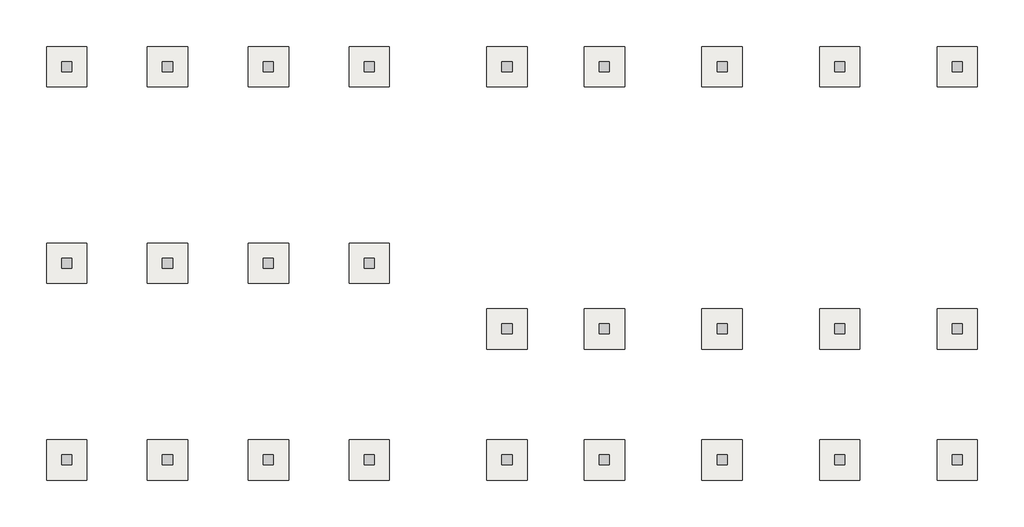
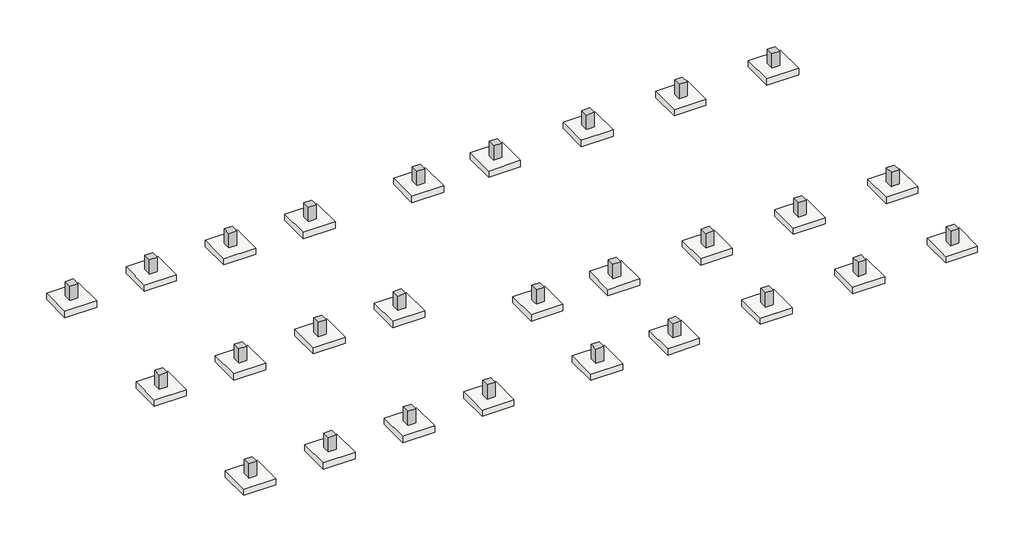
# Not in any storey: 27 columns, 27 slabs.
"""IFC4 building model written with IfcOpenShell, lengths in millimetres."""

import ifcopenshell
import ifcopenshell.guid

model = None  # the IFC model being written
_history = None  # IfcOwnerHistory: only IFC2X3 demands one
_inside = {}  # id of a spatial element -> (the spatial element, [elements in it])
_under = {}  # id of a project, library or spatial element -> (it, [spatial elements below it])
_declared = {}  # id of a project -> (the project, [libraries it declares])
_typed = {}  # id of a type object -> (the type object, [elements of that type])
_made_of = {}  # id of a material, layer set ... -> (it, [elements and type objects made of it])


def new_model(schema):
    """Start an empty IFC model of exactly this schema.

    Asked for "IFC4X3", IfcOpenShell would pick the latest addendum, in which some entities
    have other attributes; the version numbers below select the first issue.
    IFC2X3 requires an IfcOwnerHistory on every rooted entity: one is made here for all.
    """
    global model, _history
    if schema == "IFC4X3":
        model = ifcopenshell.file(schema_version=(4, 3, 0, 0))
    else:
        model = ifcopenshell.file(schema=schema)
    _inside.clear()
    _under.clear()
    _declared.clear()
    _typed.clear()
    _made_of.clear()
    _history = None
    if model.schema == "IFC2X3":
        org = make("IfcOrganization", Name="unknown")
        user = make(
            "IfcPersonAndOrganization",
            ThePerson=make("IfcPerson", FamilyName="unknown"),
            TheOrganization=org,
        )
        app = make(
            "IfcApplication",
            ApplicationDeveloper=org,
            Version="unknown",
            ApplicationFullName="unknown",
            ApplicationIdentifier="unknown",
        )
        _history = make(
            "IfcOwnerHistory",
            OwningUser=user,
            OwningApplication=app,
            ChangeAction="ADDED",
            CreationDate=0,
        )
    return model


def make(cls, **values):
    """One entity of the class cls with the attributes given. An attribute that is None is left unset."""
    return model.create_entity(
        cls, **{name: value for name, value in values.items() if value is not None}
    )


def rooted(cls, **values):
    """An entity with a GlobalId (a new one), such as an element, a storey or a relation."""
    return make(cls, GlobalId=ifcopenshell.guid.new(), OwnerHistory=_history, **values)


def si_unit(unit_type, name, prefix=None):
    """IfcSIUnit, for example si_unit("LENGTHUNIT", "METRE", prefix="MILLI")."""
    return make("IfcSIUnit", UnitType=unit_type, Prefix=prefix, Name=name)


def assignment(units):
    """IfcUnitAssignment: the units of a project."""
    return None if units is None else make("IfcUnitAssignment", Units=units)


def point(xyz):
    """IfcCartesianPoint."""
    return None if xyz is None else make("IfcCartesianPoint", Coordinates=xyz)


def direction(xyz):
    """IfcDirection."""
    return None if xyz is None else make("IfcDirection", DirectionRatios=xyz)


def frame(location, z_axis=None, x_axis=None):
    """IfcAxis2Placement3D, a coordinate frame: its origin and axes. An axis left out is left unset."""
    return make(
        "IfcAxis2Placement3D",
        Location=point(location),
        Axis=direction(z_axis),
        RefDirection=direction(x_axis),
    )


def origin():
    """The frame at (0, 0, 0) with its axes left unset."""
    return frame((0.0, 0.0, 0.0))


def place(relative_to, where):
    """IfcLocalPlacement: puts the frame where relative to a parent placement (None: the world)."""
    return make(
        "IfcLocalPlacement", PlacementRelTo=relative_to, RelativePlacement=where
    )


def context(
    kind, dimensions, precision=None, world=None, true_north=None, identifier=None
):
    """IfcGeometricRepresentationContext, for example the 3D "Model" context."""
    return make(
        "IfcGeometricRepresentationContext",
        ContextIdentifier=identifier,
        ContextType=kind,
        CoordinateSpaceDimension=dimensions,
        Precision=precision,
        WorldCoordinateSystem=world,
        TrueNorth=true_north,
    )


def project(units=None, contexts=None):
    """IfcProject with its units and contexts."""
    return rooted(
        "IfcProject",
        Name="project",
        RepresentationContexts=contexts,
        UnitsInContext=assignment(units),
    )


def spatial(cls, under=None, at=None, **own):
    """A site, building, storey or space (cls), placed at a placement, below another one or the project."""
    s = rooted(cls, ObjectPlacement=at, **own)
    if under is not None:
        _under.setdefault(under.id(), (under, []))[1].append(s)
    return s


def polyline(points):
    """IfcPolyline through the points."""
    return make("IfcPolyline", Points=[point(p) for p in points])


def outline(outer, holes=None, kind="AREA"):
    """IfcArbitraryClosedProfileDef: a profile drawn as a closed curve; with holes, ...WithVoids."""
    if holes is None:
        return make("IfcArbitraryClosedProfileDef", ProfileType=kind, OuterCurve=outer)
    return make(
        "IfcArbitraryProfileDefWithVoids",
        ProfileType=kind,
        OuterCurve=outer,
        InnerCurves=holes,
    )


def extrude(swept, where, along, depth):
    """IfcExtrudedAreaSolid: the profile swept, set in the frame where, extruded along a direction by depth."""
    return make(
        "IfcExtrudedAreaSolid",
        SweptArea=swept,
        Position=where,
        ExtrudedDirection=direction(along),
        Depth=depth,
    )


def shape(context_of_items, identifier, shape_type, items):
    """IfcShapeRepresentation: the items that make up one representation, for example the "Body"."""
    return make(
        "IfcShapeRepresentation",
        ContextOfItems=context_of_items,
        RepresentationIdentifier=identifier,
        RepresentationType=shape_type,
        Items=items,
    )


def source(mapping_origin, context_of_items, identifier, shape_type, items):
    """IfcRepresentationMap: a shape defined once, which mapped items show again and again."""
    return make(
        "IfcRepresentationMap",
        MappingOrigin=mapping_origin,
        MappedRepresentation=shape(context_of_items, identifier, shape_type, items),
    )


def transform(
    local_origin,
    x_axis=None,
    y_axis=None,
    z_axis=None,
    scale=None,
    scale2=None,
    scale3=None,
    uniform=True,
):
    """IfcCartesianTransformationOperator3D, or its non-uniform kind. x_axis, y_axis, z_axis: its Axis1, 2, 3."""
    if uniform:
        return make(
            "IfcCartesianTransformationOperator3D",
            Axis1=direction(x_axis),
            Axis2=direction(y_axis),
            LocalOrigin=point(local_origin),
            Scale=scale,
            Axis3=direction(z_axis),
        )
    return make(
        "IfcCartesianTransformationOperator3DnonUniform",
        Axis1=direction(x_axis),
        Axis2=direction(y_axis),
        LocalOrigin=point(local_origin),
        Scale=scale,
        Axis3=direction(z_axis),
        Scale2=scale2,
        Scale3=scale3,
    )


def mapped(mapping_source, mapping_target):
    """IfcMappedItem: shows the shape of a source again, moved by a transform."""
    return make(
        "IfcMappedItem", MappingSource=mapping_source, MappingTarget=mapping_target
    )


def made_of(thing, what):
    """Note that an element or type object is made of a material, layer set ...; save() writes the relation."""
    if what is not None:
        _made_of.setdefault(what.id(), (what, []))[1].append(thing)
    return thing


def element(
    cls,
    number,
    at=None,
    inside=None,
    cuts=None,
    type_object=None,
    material=None,
    context=None,
    identifier="Body",
    shape_type=None,
    held_by="IfcProductDefinitionShape",
    body=None,
    shapes=None,
    **own,
):
    """One element of the class cls, such as IfcWall. Its Tag is "e" and its number.

    at: its placement. inside: the storey or other place that contains it. cuts: it is an
    opening in that element (IfcRelVoidsElement). A single representation is given by context,
    identifier, shape_type and body (its items); several are given by shapes. held_by: the class
    of the entity that holds the representations. save() writes the other relations.
    """
    e = rooted(cls, Tag="e%d" % number, ObjectPlacement=at, **own)
    if body is not None:
        shapes = [shape(context, identifier, shape_type, body)]
    if shapes is not None:
        e.Representation = make(held_by, Representations=shapes)
    if inside is not None:
        _inside.setdefault(inside.id(), (inside, []))[1].append(e)
    if cuts is not None:
        rooted(
            "IfcRelVoidsElement", RelatingBuildingElement=cuts, RelatedOpeningElement=e
        )
    if type_object is not None:
        _typed.setdefault(type_object.id(), (type_object, []))[1].append(e)
    return made_of(e, material)


def aggregate(whole, parts):
    """IfcRelAggregates: a whole, such as a stair, and the parts it consists of."""
    return rooted("IfcRelAggregates", RelatingObject=whole, RelatedObjects=parts)


def save(model, path):
    """Write the relations noted so far, then the file.

    IfcRelAggregates (storeys below a building ...), IfcRelContainedInSpatialStructure (elements
    in a storey), IfcRelDefinesByType, IfcRelAssociatesMaterial and IfcRelDeclares: one each for
    every whole, place, type object, material and project.
    """
    for whole, parts in _under.values():
        aggregate(whole, parts)
    for where, things in _inside.values():
        rooted(
            "IfcRelContainedInSpatialStructure",
            RelatedElements=things,
            RelatingStructure=where,
        )
    for kind, things in _typed.values():
        rooted("IfcRelDefinesByType", RelatedObjects=things, RelatingType=kind)
    for what, things in _made_of.values():
        rooted("IfcRelAssociatesMaterial", RelatedObjects=things, RelatingMaterial=what)
    for by, libraries in _declared.values():
        rooted("IfcRelDeclares", RelatingContext=by, RelatedDefinitions=libraries)
    model.write(path)


def foundation_rectangular_non_pile_5fe39465(model_context):
    return source(origin(), model_context, "Body", "SweptSolid", [
        extrude(outline(polyline([(1200.0, 1200.0), (1200.0, -1200.0), (-1200.0, -1200.0), (-1200.0, 1200.0), (1200.0, 1200.0)])), frame((0.0, 0.0, -500.0), z_axis=(0.0, 0.0, 1.0), x_axis=(1.0, 0.0, 0.0)), (0.0, 0.0, 1.0), 500.0),
    ])


model = new_model("IFC4")

# Units and contexts
model_context = context("Model", 3, world=origin())
ifc_project = project(units=[si_unit("LENGTHUNIT", "METRE", prefix="MILLI")], contexts=[model_context])

# Site, building
site = spatial("IfcSite", under=ifc_project)
building = spatial("IfcBuilding", under=site)

# Columns
placement = place(None, origin())
element("IfcColumn", 1, ObjectType="RC_Column_Rectangular : H_SC_AR_S15_UG PED_W600xL600_Bit_Anchor", at=placement, inside=building, context=model_context, shape_type="SweptSolid", body=[
    extrude(outline(polyline([(300.0, 12499.5208589), (300.0, 11899.5208589), (-300.0, 11899.5208589), (-300.0, 12499.5208589), (300.0, 12499.5208589)])), frame((0.0, 0.0, -1000.0381366), z_axis=(0.0, 0.0, 1.0), x_axis=(1.0, 0.0, 0.0)), (0.0, 0.0, 1.0), 1150.0),
])
element("IfcColumn", 2, ObjectType="RC_Column_Rectangular : H_SC_AR_S15_UG PED_W600xL600_Bit_Anchor", at=placement, inside=building, context=model_context, shape_type="SweptSolid", body=[
    extrude(outline(polyline([(6300.0, 12499.5208589), (6300.0, 11899.5208589), (5700.0, 11899.5208589), (5700.0, 12499.5208589), (6300.0, 12499.5208589)])), frame((0.0, 0.0, -1000.0381366), z_axis=(0.0, 0.0, 1.0), x_axis=(1.0, 0.0, 0.0)), (0.0, 0.0, 1.0), 1150.0),
])
element("IfcColumn", 3, ObjectType="RC_Column_Rectangular : H_SC_AR_S15_UG PED_W600xL600_Bit_Anchor", at=placement, inside=building, context=model_context, shape_type="SweptSolid", body=[
    extrude(outline(polyline([(12300.0, 12499.5208589), (12300.0, 11899.5208589), (11700.0, 11899.5208589), (11700.0, 12499.5208589), (12300.0, 12499.5208589)])), frame((0.0, 0.0, -1000.0381366), z_axis=(0.0, 0.0, 1.0), x_axis=(1.0, 0.0, 0.0)), (0.0, 0.0, 1.0), 1150.0),
])
element("IfcColumn", 4, ObjectType="RC_Column_Rectangular : H_SC_AR_S15_UG PED_W600xL600_Bit_Anchor", at=placement, inside=building, context=model_context, shape_type="SweptSolid", body=[
    extrude(outline(polyline([(18300.0, 12499.5208589), (18300.0, 11899.5208589), (17700.0, 11899.5208589), (17700.0, 12499.5208589), (18300.0, 12499.5208589)])), frame((0.0, 0.0, -1000.0381366), z_axis=(0.0, 0.0, 1.0), x_axis=(1.0, 0.0, 0.0)), (0.0, 0.0, 1.0), 1150.0),
])
element("IfcColumn", 5, ObjectType="RC_Column_Rectangular : H_SC_AR_S15_UG PED_W600xL600_Bit_Anchor", at=placement, inside=building, context=model_context, shape_type="SweptSolid", body=[
    extrude(outline(polyline([(300.0, 24199.5208589), (300.0, 23599.5208589), (-300.0, 23599.5208589), (-300.0, 24199.5208589), (300.0, 24199.5208589)])), frame((0.0, 0.0, -1000.0381366), z_axis=(0.0, 0.0, 1.0), x_axis=(1.0, 0.0, 0.0)), (0.0, 0.0, 1.0), 1150.0),
])
element("IfcColumn", 6, ObjectType="RC_Column_Rectangular : H_SC_AR_S15_UG PED_W600xL600_Bit_Anchor", at=placement, inside=building, context=model_context, shape_type="SweptSolid", body=[
    extrude(outline(polyline([(6300.0, 24199.5208589), (6300.0, 23599.5208589), (5700.0, 23599.5208589), (5700.0, 24199.5208589), (6300.0, 24199.5208589)])), frame((0.0, 0.0, -1000.0381366), z_axis=(0.0, 0.0, 1.0), x_axis=(1.0, 0.0, 0.0)), (0.0, 0.0, 1.0), 1150.0),
])
element("IfcColumn", 7, ObjectType="RC_Column_Rectangular : H_SC_AR_S15_UG PED_W600xL600_Bit_Anchor", at=placement, inside=building, context=model_context, shape_type="SweptSolid", body=[
    extrude(outline(polyline([(12300.0, 24199.5208589), (12300.0, 23599.5208589), (11700.0, 23599.5208589), (11700.0, 24199.5208589), (12300.0, 24199.5208589)])), frame((0.0, 0.0, -1000.0381366), z_axis=(0.0, 0.0, 1.0), x_axis=(1.0, 0.0, 0.0)), (0.0, 0.0, 1.0), 1150.0),
])
element("IfcColumn", 8, ObjectType="RC_Column_Rectangular : H_SC_AR_S15_UG PED_W600xL600_Bit_Anchor", at=placement, inside=building, context=model_context, shape_type="SweptSolid", body=[
    extrude(outline(polyline([(18300.0, 24199.5208589), (18300.0, 23599.5208589), (17700.0, 23599.5208589), (17700.0, 24199.5208589), (18300.0, 24199.5208589)])), frame((0.0, 0.0, -1000.0381366), z_axis=(0.0, 0.0, 1.0), x_axis=(1.0, 0.0, 0.0)), (0.0, 0.0, 1.0), 1150.0),
])
element("IfcColumn", 9, ObjectType="RC_Column_Rectangular : H_SC_AR_S15_UG PED_W600xL600_Bit_Anchor", at=placement, inside=building, context=model_context, shape_type="SweptSolid", body=[
    extrude(outline(polyline([(26500.0, 24199.5208589), (26500.0, 23599.5208589), (25900.0, 23599.5208589), (25900.0, 24199.5208589), (26500.0, 24199.5208589)])), frame((0.0, 0.0, -1000.0381366), z_axis=(0.0, 0.0, 1.0), x_axis=(1.0, 0.0, 0.0)), (0.0, 0.0, 1.0), 1150.0),
])
element("IfcColumn", 10, ObjectType="RC_Column_Rectangular : H_SC_AR_S15_UG PED_W600xL600_Bit_Anchor", at=placement, inside=building, context=model_context, shape_type="SweptSolid", body=[
    extrude(outline(polyline([(32300.0, 24199.5208589), (32300.0, 23599.5208589), (31700.0, 23599.5208589), (31700.0, 24199.5208589), (32300.0, 24199.5208589)])), frame((0.0, 0.0, -1000.0381366), z_axis=(0.0, 0.0, 1.0), x_axis=(1.0, 0.0, 0.0)), (0.0, 0.0, 1.0), 1150.0),
])
element("IfcColumn", 11, ObjectType="RC_Column_Rectangular : H_SC_AR_S15_UG PED_W600xL600_Bit_Anchor", at=placement, inside=building, context=model_context, shape_type="SweptSolid", body=[
    extrude(outline(polyline([(39300.0, 24199.5208589), (39300.0, 23599.5208589), (38700.0, 23599.5208589), (38700.0, 24199.5208589), (39300.0, 24199.5208589)])), frame((0.0, 0.0, -1000.0381366), z_axis=(0.0, 0.0, 1.0), x_axis=(1.0, 0.0, 0.0)), (0.0, 0.0, 1.0), 1150.0),
])
element("IfcColumn", 12, ObjectType="RC_Column_Rectangular : H_SC_AR_S15_UG PED_W600xL600_Bit_Anchor", at=placement, inside=building, context=model_context, shape_type="SweptSolid", body=[
    extrude(outline(polyline([(46300.0, 24199.5208589), (46300.0, 23599.5208589), (45700.0, 23599.5208589), (45700.0, 24199.5208589), (46300.0, 24199.5208589)])), frame((0.0, 0.0, -1000.0381366), z_axis=(0.0, 0.0, 1.0), x_axis=(1.0, 0.0, 0.0)), (0.0, 0.0, 1.0), 1150.0),
])
element("IfcColumn", 13, ObjectType="RC_Column_Rectangular : H_SC_AR_S15_UG PED_W600xL600_Bit_Anchor", at=placement, inside=building, context=model_context, shape_type="SweptSolid", body=[
    extrude(outline(polyline([(53300.0, 24199.5208589), (53300.0, 23599.5208589), (52700.0, 23599.5208589), (52700.0, 24199.5208589), (53300.0, 24199.5208589)])), frame((0.0, 0.0, -1000.0381366), z_axis=(0.0, 0.0, 1.0), x_axis=(1.0, 0.0, 0.0)), (0.0, 0.0, 1.0), 1150.0),
])
element("IfcColumn", 14, ObjectType="RC_Column_Rectangular : H_SC_AR_S15_UG PED_W600xL600_Bit_Anchor", at=placement, inside=building, context=model_context, shape_type="SweptSolid", body=[
    extrude(outline(polyline([(26500.0, 8599.5208589), (26500.0, 7999.5208589), (25900.0, 7999.5208589), (25900.0, 8599.5208589), (26500.0, 8599.5208589)])), frame((0.0, 0.0, -1000.0381366), z_axis=(0.0, 0.0, 1.0), x_axis=(1.0, 0.0, 0.0)), (0.0, 0.0, 1.0), 1150.0),
])
element("IfcColumn", 15, ObjectType="RC_Column_Rectangular : H_SC_AR_S15_UG PED_W600xL600_Bit_Anchor", at=placement, inside=building, context=model_context, shape_type="SweptSolid", body=[
    extrude(outline(polyline([(32300.0, 8599.5208589), (32300.0, 7999.5208589), (31700.0, 7999.5208589), (31700.0, 8599.5208589), (32300.0, 8599.5208589)])), frame((0.0, 0.0, -1000.0381366), z_axis=(0.0, 0.0, 1.0), x_axis=(1.0, 0.0, 0.0)), (0.0, 0.0, 1.0), 1150.0),
])
element("IfcColumn", 16, ObjectType="RC_Column_Rectangular : H_SC_AR_S15_UG PED_W600xL600_Bit_Anchor", at=placement, inside=building, context=model_context, shape_type="SweptSolid", body=[
    extrude(outline(polyline([(39300.0, 8599.5208589), (39300.0, 7999.5208589), (38700.0, 7999.5208589), (38700.0, 8599.5208589), (39300.0, 8599.5208589)])), frame((0.0, 0.0, -1000.0381366), z_axis=(0.0, 0.0, 1.0), x_axis=(1.0, 0.0, 0.0)), (0.0, 0.0, 1.0), 1150.0),
])
element("IfcColumn", 17, ObjectType="RC_Column_Rectangular : H_SC_AR_S15_UG PED_W600xL600_Bit_Anchor", at=placement, inside=building, context=model_context, shape_type="SweptSolid", body=[
    extrude(outline(polyline([(46300.0, 8599.5208589), (46300.0, 7999.5208589), (45700.0, 7999.5208589), (45700.0, 8599.5208589), (46300.0, 8599.5208589)])), frame((0.0, 0.0, -1000.0381366), z_axis=(0.0, 0.0, 1.0), x_axis=(1.0, 0.0, 0.0)), (0.0, 0.0, 1.0), 1150.0),
])
element("IfcColumn", 18, ObjectType="RC_Column_Rectangular : H_SC_AR_S15_UG PED_W600xL600_Bit_Anchor", at=placement, inside=building, context=model_context, shape_type="SweptSolid", body=[
    extrude(outline(polyline([(53300.0, 8599.5208589), (53300.0, 7999.5208589), (52700.0, 7999.5208589), (52700.0, 8599.5208589), (53300.0, 8599.5208589)])), frame((0.0, 0.0, -1000.0381366), z_axis=(0.0, 0.0, 1.0), x_axis=(1.0, 0.0, 0.0)), (0.0, 0.0, 1.0), 1150.0),
])
element("IfcColumn", 19, ObjectType="RC_Column_Rectangular : H_SC_AR_S15_UG PED_W600xL600_Bit_Anchor", at=placement, inside=building, context=model_context, shape_type="SweptSolid", body=[
    extrude(outline(polyline([(300.0, 799.5208589), (300.0, 199.5208589), (-300.0, 199.5208589), (-300.0, 799.5208589), (300.0, 799.5208589)])), frame((0.0, 0.0, -1000.0381366), z_axis=(0.0, 0.0, 1.0), x_axis=(1.0, 0.0, 0.0)), (0.0, 0.0, 1.0), 1150.0),
])
element("IfcColumn", 20, ObjectType="RC_Column_Rectangular : H_SC_AR_S15_UG PED_W600xL600_Bit_Anchor", at=placement, inside=building, context=model_context, shape_type="SweptSolid", body=[
    extrude(outline(polyline([(6300.0, 799.5208589), (6300.0, 199.5208589), (5700.0, 199.5208589), (5700.0, 799.5208589), (6300.0, 799.5208589)])), frame((0.0, 0.0, -1000.0381366), z_axis=(0.0, 0.0, 1.0), x_axis=(1.0, 0.0, 0.0)), (0.0, 0.0, 1.0), 1150.0),
])
element("IfcColumn", 21, ObjectType="RC_Column_Rectangular : H_SC_AR_S15_UG PED_W600xL600_Bit_Anchor", at=placement, inside=building, context=model_context, shape_type="SweptSolid", body=[
    extrude(outline(polyline([(12300.0, 799.5208589), (12300.0, 199.5208589), (11700.0, 199.5208589), (11700.0, 799.5208589), (12300.0, 799.5208589)])), frame((0.0, 0.0, -1000.0381366), z_axis=(0.0, 0.0, 1.0), x_axis=(1.0, 0.0, 0.0)), (0.0, 0.0, 1.0), 1150.0),
])
element("IfcColumn", 22, ObjectType="RC_Column_Rectangular : H_SC_AR_S15_UG PED_W600xL600_Bit_Anchor", at=placement, inside=building, context=model_context, shape_type="SweptSolid", body=[
    extrude(outline(polyline([(18300.0, 799.5208589), (18300.0, 199.5208589), (17700.0, 199.5208589), (17700.0, 799.5208589), (18300.0, 799.5208589)])), frame((0.0, 0.0, -1000.0381366), z_axis=(0.0, 0.0, 1.0), x_axis=(1.0, 0.0, 0.0)), (0.0, 0.0, 1.0), 1150.0),
])
element("IfcColumn", 23, ObjectType="RC_Column_Rectangular : H_SC_AR_S15_UG PED_W600xL600_Bit_Anchor", at=placement, inside=building, context=model_context, shape_type="SweptSolid", body=[
    extrude(outline(polyline([(26500.0, 799.5208589), (26500.0, 199.5208589), (25900.0, 199.5208589), (25900.0, 799.5208589), (26500.0, 799.5208589)])), frame((0.0, 0.0, -1000.0381366), z_axis=(0.0, 0.0, 1.0), x_axis=(1.0, 0.0, 0.0)), (0.0, 0.0, 1.0), 1150.0),
])
element("IfcColumn", 24, ObjectType="RC_Column_Rectangular : H_SC_AR_S15_UG PED_W600xL600_Bit_Anchor", at=placement, inside=building, context=model_context, shape_type="SweptSolid", body=[
    extrude(outline(polyline([(32300.0, 799.5208589), (32300.0, 199.5208589), (31700.0, 199.5208589), (31700.0, 799.5208589), (32300.0, 799.5208589)])), frame((0.0, 0.0, -1000.0381366), z_axis=(0.0, 0.0, 1.0), x_axis=(1.0, 0.0, 0.0)), (0.0, 0.0, 1.0), 1150.0),
])
element("IfcColumn", 25, ObjectType="RC_Column_Rectangular : H_SC_AR_S15_UG PED_W600xL600_Bit_Anchor", at=placement, inside=building, context=model_context, shape_type="SweptSolid", body=[
    extrude(outline(polyline([(39300.0, 799.5208589), (39300.0, 199.5208589), (38700.0, 199.5208589), (38700.0, 799.5208589), (39300.0, 799.5208589)])), frame((0.0, 0.0, -1000.0381366), z_axis=(0.0, 0.0, 1.0), x_axis=(1.0, 0.0, 0.0)), (0.0, 0.0, 1.0), 1150.0),
])
element("IfcColumn", 26, ObjectType="RC_Column_Rectangular : H_SC_AR_S15_UG PED_W600xL600_Bit_Anchor", at=placement, inside=building, context=model_context, shape_type="SweptSolid", body=[
    extrude(outline(polyline([(46300.0, 799.5208589), (46300.0, 199.5208589), (45700.0, 199.5208589), (45700.0, 799.5208589), (46300.0, 799.5208589)])), frame((0.0, 0.0, -1000.0381366), z_axis=(0.0, 0.0, 1.0), x_axis=(1.0, 0.0, 0.0)), (0.0, 0.0, 1.0), 1150.0),
])
element("IfcColumn", 27, ObjectType="RC_Column_Rectangular : H_SC_AR_S15_UG PED_W600xL600_Bit_Anchor", at=placement, inside=building, context=model_context, shape_type="SweptSolid", body=[
    extrude(outline(polyline([(53300.0, 799.5208589), (53300.0, 199.5208589), (52700.0, 199.5208589), (52700.0, 799.5208589), (53300.0, 799.5208589)])), frame((0.0, 0.0, -1000.0381366), z_axis=(0.0, 0.0, 1.0), x_axis=(1.0, 0.0, 0.0)), (0.0, 0.0, 1.0), 1150.0),
])

# Slabs
foundation_rectangular_non_pile_shape = foundation_rectangular_non_pile_5fe39465(model_context)
element("IfcSlab", 28, ObjectType="Foundation Rectangular (Non-Pile) : H_SF_AR_S18_W2400xL2400xT500_Bitumen", at=placement, inside=building, context=model_context, shape_type="MappedRepresentation", body=[
    mapped(foundation_rectangular_non_pile_shape, transform((0.0, 12199.5208589, -1000.0381366), x_axis=(1.0, 0.0, 0.0), y_axis=(0.0, 1.0, 0.0), z_axis=(0.0, 0.0, 1.0))),
])
element("IfcSlab", 29, ObjectType="Foundation Rectangular (Non-Pile) : H_SF_AR_S18_W2400xL2400xT500_Bitumen", at=placement, inside=building, context=model_context, shape_type="MappedRepresentation", body=[
    mapped(foundation_rectangular_non_pile_shape, transform((6000.0, 12199.5208589, -1000.0381366), x_axis=(1.0, 0.0, 0.0), y_axis=(0.0, 1.0, 0.0), z_axis=(0.0, 0.0, 1.0))),
])
element("IfcSlab", 30, ObjectType="Foundation Rectangular (Non-Pile) : H_SF_AR_S18_W2400xL2400xT500_Bitumen", at=placement, inside=building, context=model_context, shape_type="MappedRepresentation", body=[
    mapped(foundation_rectangular_non_pile_shape, transform((12000.0, 12199.5208589, -1000.0381366), x_axis=(1.0, 0.0, 0.0), y_axis=(0.0, 1.0, 0.0), z_axis=(0.0, 0.0, 1.0))),
])
element("IfcSlab", 31, ObjectType="Foundation Rectangular (Non-Pile) : H_SF_AR_S18_W2400xL2400xT500_Bitumen", at=placement, inside=building, context=model_context, shape_type="MappedRepresentation", body=[
    mapped(foundation_rectangular_non_pile_shape, transform((18000.0, 12199.5208589, -1000.0381366), x_axis=(1.0, 0.0, 0.0), y_axis=(0.0, 1.0, 0.0), z_axis=(0.0, 0.0, 1.0))),
])
element("IfcSlab", 32, ObjectType="Foundation Rectangular (Non-Pile) : H_SF_AR_S18_W2400xL2400xT500_Bitumen", at=placement, inside=building, context=model_context, shape_type="MappedRepresentation", body=[
    mapped(foundation_rectangular_non_pile_shape, transform((0.0, 23899.5208589, -1000.0381366), x_axis=(1.0, 0.0, 0.0), y_axis=(0.0, 1.0, 0.0), z_axis=(0.0, 0.0, 1.0))),
])
element("IfcSlab", 33, ObjectType="Foundation Rectangular (Non-Pile) : H_SF_AR_S18_W2400xL2400xT500_Bitumen", at=placement, inside=building, context=model_context, shape_type="MappedRepresentation", body=[
    mapped(foundation_rectangular_non_pile_shape, transform((6000.0, 23899.5208589, -1000.0381366), x_axis=(1.0, 0.0, 0.0), y_axis=(0.0, 1.0, 0.0), z_axis=(0.0, 0.0, 1.0))),
])
element("IfcSlab", 34, ObjectType="Foundation Rectangular (Non-Pile) : H_SF_AR_S18_W2400xL2400xT500_Bitumen", at=placement, inside=building, context=model_context, shape_type="MappedRepresentation", body=[
    mapped(foundation_rectangular_non_pile_shape, transform((12000.0, 23899.5208589, -1000.0381366), x_axis=(1.0, 0.0, 0.0), y_axis=(0.0, 1.0, 0.0), z_axis=(0.0, 0.0, 1.0))),
])
element("IfcSlab", 35, ObjectType="Foundation Rectangular (Non-Pile) : H_SF_AR_S18_W2400xL2400xT500_Bitumen", at=placement, inside=building, context=model_context, shape_type="MappedRepresentation", body=[
    mapped(foundation_rectangular_non_pile_shape, transform((18000.0, 23899.5208589, -1000.0381366), x_axis=(1.0, 0.0, 0.0), y_axis=(0.0, 1.0, 0.0), z_axis=(0.0, 0.0, 1.0))),
])
element("IfcSlab", 36, ObjectType="Foundation Rectangular (Non-Pile) : H_SF_AR_S18_W2400xL2400xT500_Bitumen", at=placement, inside=building, context=model_context, shape_type="MappedRepresentation", body=[
    mapped(foundation_rectangular_non_pile_shape, transform((26200.0, 23899.5208589, -1000.0381366), x_axis=(1.0, 0.0, 0.0), y_axis=(0.0, 1.0, 0.0), z_axis=(0.0, 0.0, 1.0))),
])
element("IfcSlab", 37, ObjectType="Foundation Rectangular (Non-Pile) : H_SF_AR_S18_W2400xL2400xT500_Bitumen", at=placement, inside=building, context=model_context, shape_type="MappedRepresentation", body=[
    mapped(foundation_rectangular_non_pile_shape, transform((32000.0, 23899.5208589, -1000.0381366), x_axis=(1.0, 0.0, 0.0), y_axis=(0.0, 1.0, 0.0), z_axis=(0.0, 0.0, 1.0))),
])
element("IfcSlab", 38, ObjectType="Foundation Rectangular (Non-Pile) : H_SF_AR_S18_W2400xL2400xT500_Bitumen", at=placement, inside=building, context=model_context, shape_type="MappedRepresentation", body=[
    mapped(foundation_rectangular_non_pile_shape, transform((39000.0, 23899.5208589, -1000.0381366), x_axis=(1.0, 0.0, 0.0), y_axis=(0.0, 1.0, 0.0), z_axis=(0.0, 0.0, 1.0))),
])
element("IfcSlab", 39, ObjectType="Foundation Rectangular (Non-Pile) : H_SF_AR_S18_W2400xL2400xT500_Bitumen", at=placement, inside=building, context=model_context, shape_type="MappedRepresentation", body=[
    mapped(foundation_rectangular_non_pile_shape, transform((46000.0, 23899.5208589, -1000.0381366), x_axis=(1.0, 0.0, 0.0), y_axis=(0.0, 1.0, 0.0), z_axis=(0.0, 0.0, 1.0))),
])
element("IfcSlab", 40, ObjectType="Foundation Rectangular (Non-Pile) : H_SF_AR_S18_W2400xL2400xT500_Bitumen", at=placement, inside=building, context=model_context, shape_type="MappedRepresentation", body=[
    mapped(foundation_rectangular_non_pile_shape, transform((53000.0, 23899.5208589, -1000.0381366), x_axis=(1.0, 0.0, 0.0), y_axis=(0.0, 1.0, 0.0), z_axis=(0.0, 0.0, 1.0))),
])
element("IfcSlab", 41, ObjectType="Foundation Rectangular (Non-Pile) : H_SF_AR_S18_W2400xL2400xT500_Bitumen", at=placement, inside=building, context=model_context, shape_type="MappedRepresentation", body=[
    mapped(foundation_rectangular_non_pile_shape, transform((26200.0, 8299.5208589, -1000.0381366), x_axis=(1.0, 0.0, 0.0), y_axis=(0.0, 1.0, 0.0), z_axis=(0.0, 0.0, 1.0))),
])
element("IfcSlab", 42, ObjectType="Foundation Rectangular (Non-Pile) : H_SF_AR_S18_W2400xL2400xT500_Bitumen", at=placement, inside=building, context=model_context, shape_type="MappedRepresentation", body=[
    mapped(foundation_rectangular_non_pile_shape, transform((32000.0, 8299.5208589, -1000.0381366), x_axis=(1.0, 0.0, 0.0), y_axis=(0.0, 1.0, 0.0), z_axis=(0.0, 0.0, 1.0))),
])
element("IfcSlab", 43, ObjectType="Foundation Rectangular (Non-Pile) : H_SF_AR_S18_W2400xL2400xT500_Bitumen", at=placement, inside=building, context=model_context, shape_type="MappedRepresentation", body=[
    mapped(foundation_rectangular_non_pile_shape, transform((39000.0, 8299.5208589, -1000.0381366), x_axis=(1.0, 0.0, 0.0), y_axis=(0.0, 1.0, 0.0), z_axis=(0.0, 0.0, 1.0))),
])
element("IfcSlab", 44, ObjectType="Foundation Rectangular (Non-Pile) : H_SF_AR_S18_W2400xL2400xT500_Bitumen", at=placement, inside=building, context=model_context, shape_type="MappedRepresentation", body=[
    mapped(foundation_rectangular_non_pile_shape, transform((46000.0, 8299.5208589, -1000.0381366), x_axis=(1.0, 0.0, 0.0), y_axis=(0.0, 1.0, 0.0), z_axis=(0.0, 0.0, 1.0))),
])
element("IfcSlab", 45, ObjectType="Foundation Rectangular (Non-Pile) : H_SF_AR_S18_W2400xL2400xT500_Bitumen", at=placement, inside=building, context=model_context, shape_type="MappedRepresentation", body=[
    mapped(foundation_rectangular_non_pile_shape, transform((53000.0, 8299.5208589, -1000.0381366), x_axis=(1.0, 0.0, 0.0), y_axis=(0.0, 1.0, 0.0), z_axis=(0.0, 0.0, 1.0))),
])
element("IfcSlab", 46, ObjectType="Foundation Rectangular (Non-Pile) : H_SF_AR_S18_W2400xL2400xT500_Bitumen", at=placement, inside=building, context=model_context, shape_type="MappedRepresentation", body=[
    mapped(foundation_rectangular_non_pile_shape, transform((0.0, 499.5208589, -1000.0381366), x_axis=(1.0, 0.0, 0.0), y_axis=(0.0, 1.0, 0.0), z_axis=(0.0, 0.0, 1.0))),
])
element("IfcSlab", 47, ObjectType="Foundation Rectangular (Non-Pile) : H_SF_AR_S18_W2400xL2400xT500_Bitumen", at=placement, inside=building, context=model_context, shape_type="MappedRepresentation", body=[
    mapped(foundation_rectangular_non_pile_shape, transform((6000.0, 499.5208589, -1000.0381366), x_axis=(1.0, 0.0, 0.0), y_axis=(0.0, 1.0, 0.0), z_axis=(0.0, 0.0, 1.0))),
])
element("IfcSlab", 48, ObjectType="Foundation Rectangular (Non-Pile) : H_SF_AR_S18_W2400xL2400xT500_Bitumen", at=placement, inside=building, context=model_context, shape_type="MappedRepresentation", body=[
    mapped(foundation_rectangular_non_pile_shape, transform((12000.0, 499.5208589, -1000.0381366), x_axis=(1.0, 0.0, 0.0), y_axis=(0.0, 1.0, 0.0), z_axis=(0.0, 0.0, 1.0))),
])
element("IfcSlab", 49, ObjectType="Foundation Rectangular (Non-Pile) : H_SF_AR_S18_W2400xL2400xT500_Bitumen", at=placement, inside=building, context=model_context, shape_type="MappedRepresentation", body=[
    mapped(foundation_rectangular_non_pile_shape, transform((18000.0, 499.5208589, -1000.0381366), x_axis=(1.0, 0.0, 0.0), y_axis=(0.0, 1.0, 0.0), z_axis=(0.0, 0.0, 1.0))),
])
element("IfcSlab", 50, ObjectType="Foundation Rectangular (Non-Pile) : H_SF_AR_S18_W2400xL2400xT500_Bitumen", at=placement, inside=building, context=model_context, shape_type="MappedRepresentation", body=[
    mapped(foundation_rectangular_non_pile_shape, transform((26200.0, 499.5208589, -1000.0381366), x_axis=(1.0, 0.0, 0.0), y_axis=(0.0, 1.0, 0.0), z_axis=(0.0, 0.0, 1.0))),
])
element("IfcSlab", 51, ObjectType="Foundation Rectangular (Non-Pile) : H_SF_AR_S18_W2400xL2400xT500_Bitumen", at=placement, inside=building, context=model_context, shape_type="MappedRepresentation", body=[
    mapped(foundation_rectangular_non_pile_shape, transform((32000.0, 499.5208589, -1000.0381366), x_axis=(1.0, 0.0, 0.0), y_axis=(0.0, 1.0, 0.0), z_axis=(0.0, 0.0, 1.0))),
])
element("IfcSlab", 52, ObjectType="Foundation Rectangular (Non-Pile) : H_SF_AR_S18_W2400xL2400xT500_Bitumen", at=placement, inside=building, context=model_context, shape_type="MappedRepresentation", body=[
    mapped(foundation_rectangular_non_pile_shape, transform((39000.0, 499.5208589, -1000.0381366), x_axis=(1.0, 0.0, 0.0), y_axis=(0.0, 1.0, 0.0), z_axis=(0.0, 0.0, 1.0))),
])
element("IfcSlab", 53, ObjectType="Foundation Rectangular (Non-Pile) : H_SF_AR_S18_W2400xL2400xT500_Bitumen", at=placement, inside=building, context=model_context, shape_type="MappedRepresentation", body=[
    mapped(foundation_rectangular_non_pile_shape, transform((46000.0, 499.5208589, -1000.0381366), x_axis=(1.0, 0.0, 0.0), y_axis=(0.0, 1.0, 0.0), z_axis=(0.0, 0.0, 1.0))),
])
element("IfcSlab", 54, ObjectType="Foundation Rectangular (Non-Pile) : H_SF_AR_S18_W2400xL2400xT500_Bitumen", at=placement, inside=building, context=model_context, shape_type="MappedRepresentation", body=[
    mapped(foundation_rectangular_non_pile_shape, transform((53000.0, 499.5208589, -1000.0381366), x_axis=(1.0, 0.0, 0.0), y_axis=(0.0, 1.0, 0.0), z_axis=(0.0, 0.0, 1.0))),
])

save(model, "model.ifc")

# Revit data of these elements
# Type "RC_Column_Rectangular : H_SC_AR_S15_UG PED_W600xL600_Bit_Anchor"
#   Width = 600 mm
#   Length = 600 mm
#   hec_material3 [instance default] = none
#   hec_material2 [instance default] = none
#   hec_material1 [instance default] = none
#   Structural Material [instance default] = none
#   Description = (empty or 0)
# Type "Foundation Rectangular (Non-Pile) : H_SF_AR_S18_W2400xL2400xT500_Bitumen"
#   Top bar = "D25@300"
#   Description = "UG Shallow Foundation"
#   Bottom bar = "D20@300"
#   Width = 2400 mm
#   Length = 2400 mm
#   Foundation Thickness = 500 mm
#   Structural Material [instance default] = none
#   Assembly Code = ""
# Elements 1, 2, 3, 4, 5, 6, 7, 8, 9, 10, 11, 12, 13, 14, 15, 16, 17, 18, 19, 20, 21, 22, 23, 24, 25, 26, 27 (IfcColumn, "RC_Column_Rectangular : H_SC_AR_S15_UG PED_W600xL600_Bit_Anchor")
#   Comments = ""
#   hec_material3 = none
#   hec_material2 = none
#   hec_material1 = none
#   Structural Material = none
#   Phase Created = New Construction
# Elements 28, 29, 30, 31, 32, 33, 34, 35, 36, 37, 38, 39, 40, 41, 42, 43, 44, 45, 46, 47, 48, 49, 50, 51, 52, 53, 54 (IfcSlab, "Foundation Rectangular (Non-Pile) : H_SF_AR_S18_W2400xL2400xT500_Bitumen")
#   Comments = ""
#   Structural Material = none
#   Phase Created = New Construction
